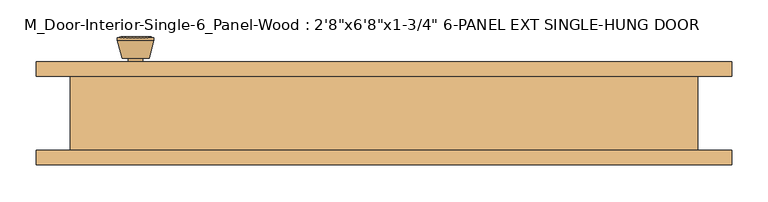
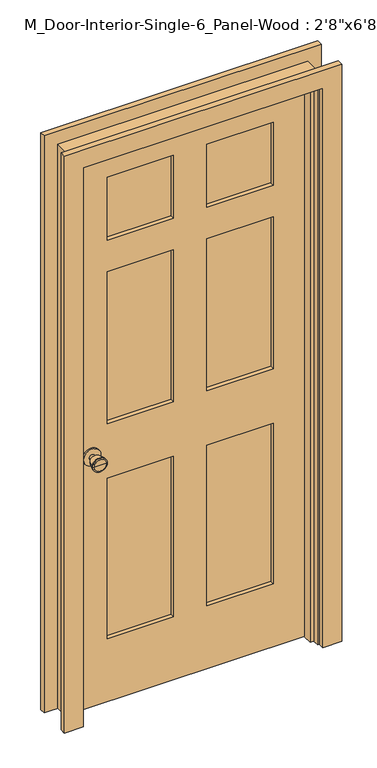
"""IFC4 building model written with IfcOpenShell, lengths in millimetres: door geometry."""

from ifc_helpers import new_model, si_unit, point, frame, frame_2d, origin, place, context, project, spatial, polyline, circle_curve, trimmed, segment, composite_curve, outline, extrude, faceted_brep, source, transform, mapped, element, save
from ifc_brep_helpers import plane_surface, cylinder_surface, revolved_surface, advanced_brep


def door_1e006c27(model_context):
    return source(origin(), model_context, "Body", "SolidModel", [
        advanced_brep(
        [(-341.4, -2.825, 914.4), (-331.4, -2.825, 914.4), (-351.4, -2.825, 914.4), (-320.9241324, -51.825, 914.4), (-341.4, -51.825, 914.4), (-361.8758676, -51.825, 914.4), (-316.4, -49.9971319, 914.4), (-366.4, -49.9971319, 914.4), (-316.4, -46.5334537, 914.4), (-366.4, -46.5334537, 914.4), (-322.763764, -21.825, 914.4), (-360.036236, -21.825, 914.4), (-331.4, -21.825, 914.4), (-351.4, -21.825, 914.4)],
        [
            (0, 1),
            (1, 2, circle_curve(frame((-341.4, -2.825, 914.4), z_axis=(0.0, 1.0, 0.0), x_axis=(-1.0, 0.0, 0.0)), 10.0)),
            (2, 0),
            (2, 1, circle_curve(frame((-341.4, -2.825, 914.4), z_axis=(0.0, 1.0, 0.0), x_axis=(-1.0, 0.0, 0.0)), 10.0)),
            (3, 4),
            (4, 5),
            (5, 3, circle_curve(frame((-341.4, -51.825, 914.4), z_axis=(0.0, -1.0, 0.0), x_axis=(-1.0, 0.0, 0.0)), 20.4758676)),
            (3, 5, circle_curve(frame((-341.4, -51.825, 914.4), z_axis=(0.0, -1.0, 0.0), x_axis=(-1.0, 0.0, 0.0)), 20.4758676)),
            (6, 3),
            (5, 7),
            (7, 6, circle_curve(frame((-341.4, -49.9971319, 914.4), z_axis=(0.0, -1.0, 0.0), x_axis=(-1.0, 0.0, 0.0)), 25.0)),
            (6, 7, circle_curve(frame((-341.4, -49.9971319, 914.4), z_axis=(0.0, -1.0, 0.0), x_axis=(-1.0, 0.0, 0.0)), 25.0)),
            (8, 6),
            (7, 9),
            (9, 8, circle_curve(frame((-341.4, -46.5334537, 914.4), z_axis=(0.0, -1.0, 0.0), x_axis=(-1.0, 0.0, 0.0)), 25.0)),
            (8, 9, circle_curve(frame((-341.4, -46.5334537, 914.4), z_axis=(0.0, -1.0, 0.0), x_axis=(-1.0, 0.0, 0.0)), 25.0)),
            (10, 8),
            (9, 11),
            (11, 10, circle_curve(frame((-341.4, -21.825, 914.4), z_axis=(0.0, -1.0, 0.0), x_axis=(-1.0, 0.0, 0.0)), 18.636236)),
            (10, 11, circle_curve(frame((-341.4, -21.825, 914.4), z_axis=(0.0, -1.0, 0.0), x_axis=(-1.0, 0.0, 0.0)), 18.636236)),
            (12, 10),
            (11, 13),
            (13, 12, circle_curve(frame((-341.4, -21.825, 914.4), z_axis=(0.0, -1.0, 0.0), x_axis=(-1.0, 0.0, 0.0)), 10.0)),
            (12, 13, circle_curve(frame((-341.4, -21.825, 914.4), z_axis=(0.0, -1.0, 0.0), x_axis=(-1.0, 0.0, 0.0)), 10.0)),
            (1, 12),
            (13, 2),
        ],
        [
            plane_surface(frame((-341.4, -2.825, 914.4), z_axis=(0.0, 1.0, 0.0), x_axis=(-1.0, 0.0, 0.0))),
            plane_surface(frame((-341.4, -51.825, 914.4), z_axis=(0.0, -1.0, 0.0), x_axis=(-1.0, 0.0, 0.0))),
            revolved_surface(polyline([(-361.8758676, -51.825, 914.4), (-366.4, -49.9971319, 914.4)]), (-341.4, -2.825, 914.4), (0.0, 1.0, 0.0)),
            cylinder_surface(frame((-341.4, -2.825, 914.4), z_axis=(0.0, 1.0, 0.0), x_axis=(-1.0, 0.0, 0.0)), 25.0),
            revolved_surface(polyline([(-366.4, -46.5334537, 914.4), (-360.036236, -21.825, 914.4)]), (-341.4, -2.825, 914.4), (0.0, 1.0, 0.0)),
            plane_surface(frame((-341.4, -21.825, 914.4), z_axis=(0.0, 1.0, 0.0), x_axis=(-1.0, 0.0, 0.0))),
            cylinder_surface(frame((-341.4, -2.825, 914.4), z_axis=(0.0, 1.0, 0.0), x_axis=(-1.0, 0.0, 0.0)), 10.0),
        ],
        [
            (0, [[1, 2, 3]]),
            (0, [[-3, 4, -1]]),
            (1, [[5, 6, 7]]),
            (1, [[-6, -5, 8]]),
            (2, [[9, -7, 10, 11]]),
            (2, [[-10, -8, -9, 12]]),
            (3, [[13, -11, 14, 15]]),
            (3, [[-14, -12, -13, 16]]),
            (4, [[17, -15, 18, 19]]),
            (4, [[-18, -16, -17, 20]]),
            (5, [[21, -19, 22, 23]]),
            (5, [[-22, -20, -21, 24]]),
            (6, [[25, -23, 26, -2]]),
            (6, [[-26, -24, -25, -4]]),
        ],
    ),
        extrude(outline(composite_curve([segment(trimmed(circle_curve(frame_2d((914.4, -341.4)), 30.0), [point((914.4, -371.4))], [point((914.4, -311.4))], False, "CARTESIAN"), True, "CONTINUOUS"), segment(trimmed(circle_curve(frame_2d((914.4, -341.4)), 30.0), [point((914.4, -311.4))], [point((914.4, -371.4))], False, "CARTESIAN"), True, "CONTINUOUS")], self_intersect=False)), frame((0.0, -2.825, 0.0), z_axis=(0.0, 1.0, 0.0), x_axis=(0.0, 0.0, 1.0)), (0.0, 0.0, 1.0), 6.0),
        advanced_brep(
        [(-341.4, 53.625, 914.4), (-351.4, 53.625, 914.4), (-331.4, 53.625, 914.4), (-320.9241324, 102.625, 914.4), (-361.8758676, 102.625, 914.4), (-341.4, 102.625, 914.4), (-316.4, 100.7971319, 914.4), (-366.4, 100.7971319, 914.4), (-316.4, 97.3334537, 914.4), (-366.4, 97.3334537, 914.4), (-322.763764, 72.625, 914.4), (-360.036236, 72.625, 914.4), (-331.4, 72.625, 914.4), (-351.4, 72.625, 914.4)],
        [
            (0, 1),
            (1, 2, circle_curve(frame((-341.4, 53.625, 914.4), z_axis=(0.0, -1.0, 0.0), x_axis=(-1.0, 0.0, 0.0)), 10.0)),
            (2, 0),
            (2, 1, circle_curve(frame((-341.4, 53.625, 914.4), z_axis=(0.0, -1.0, 0.0), x_axis=(-1.0, 0.0, 0.0)), 10.0)),
            (3, 4, circle_curve(frame((-341.4, 102.625, 914.4), z_axis=(0.0, 1.0, 0.0), x_axis=(-1.0, 0.0, 0.0)), 20.4758676)),
            (4, 5),
            (5, 3),
            (4, 3, circle_curve(frame((-341.4, 102.625, 914.4), z_axis=(0.0, 1.0, 0.0), x_axis=(-1.0, 0.0, 0.0)), 20.4758676)),
            (6, 7, circle_curve(frame((-341.4, 100.7971319, 914.4), z_axis=(0.0, 1.0, 0.0), x_axis=(-1.0, 0.0, 0.0)), 25.0)),
            (7, 4),
            (3, 6),
            (7, 6, circle_curve(frame((-341.4, 100.7971319, 914.4), z_axis=(0.0, 1.0, 0.0), x_axis=(-1.0, 0.0, 0.0)), 25.0)),
            (8, 9, circle_curve(frame((-341.4, 97.3334537, 914.4), z_axis=(0.0, 1.0, 0.0), x_axis=(-1.0, 0.0, 0.0)), 25.0)),
            (9, 7),
            (6, 8),
            (9, 8, circle_curve(frame((-341.4, 97.3334537, 914.4), z_axis=(0.0, 1.0, 0.0), x_axis=(-1.0, 0.0, 0.0)), 25.0)),
            (10, 11, circle_curve(frame((-341.4, 72.625, 914.4), z_axis=(0.0, 1.0, 0.0), x_axis=(-1.0, 0.0, 0.0)), 18.636236)),
            (11, 9),
            (8, 10),
            (11, 10, circle_curve(frame((-341.4, 72.625, 914.4), z_axis=(0.0, 1.0, 0.0), x_axis=(-1.0, 0.0, 0.0)), 18.636236)),
            (12, 13, circle_curve(frame((-341.4, 72.625, 914.4), z_axis=(0.0, 1.0, 0.0), x_axis=(-1.0, 0.0, 0.0)), 10.0)),
            (13, 11),
            (10, 12),
            (13, 12, circle_curve(frame((-341.4, 72.625, 914.4), z_axis=(0.0, 1.0, 0.0), x_axis=(-1.0, 0.0, 0.0)), 10.0)),
            (1, 13),
            (12, 2),
        ],
        [
            plane_surface(frame((-341.4, 53.625, 914.4), z_axis=(0.0, -1.0, 0.0), x_axis=(-1.0, 0.0, 0.0))),
            plane_surface(frame((-341.4, 102.625, 914.4), z_axis=(0.0, 1.0, 0.0), x_axis=(-1.0, 0.0, 0.0))),
            revolved_surface(polyline([(-361.8758676, 102.625, 914.4), (-366.4, 100.7971319, 914.4)]), (-341.4, 53.625, 914.4), (0.0, -1.0, 0.0)),
            cylinder_surface(frame((-341.4, 53.625, 914.4), z_axis=(0.0, -1.0, 0.0), x_axis=(-1.0, 0.0, 0.0)), 25.0),
            revolved_surface(polyline([(-366.4, 97.3334537, 914.4), (-360.036236, 72.625, 914.4)]), (-341.4, 53.625, 914.4), (0.0, -1.0, 0.0)),
            plane_surface(frame((-341.4, 72.625, 914.4), z_axis=(0.0, -1.0, 0.0), x_axis=(-1.0, 0.0, 0.0))),
            cylinder_surface(frame((-341.4, 53.625, 914.4), z_axis=(0.0, -1.0, 0.0), x_axis=(-1.0, 0.0, 0.0)), 10.0),
        ],
        [
            (0, [[1, 2, 3]]),
            (0, [[-3, 4, -1]]),
            (1, [[5, 6, 7]]),
            (1, [[8, -7, -6]]),
            (2, [[9, 10, -5, 11]]),
            (2, [[12, -11, -8, -10]]),
            (3, [[13, 14, -9, 15]]),
            (3, [[16, -15, -12, -14]]),
            (4, [[17, 18, -13, 19]]),
            (4, [[20, -19, -16, -18]]),
            (5, [[21, 22, -17, 23]]),
            (5, [[24, -23, -20, -22]]),
            (6, [[-2, 25, -21, 26]]),
            (6, [[-4, -26, -24, -25]]),
        ],
    ),
        extrude(outline(composite_curve([segment(trimmed(circle_curve(frame_2d((914.4, -341.4)), 30.0), [point((914.4, -371.4))], [point((914.4, -311.4))], False, "CARTESIAN"), True, "CONTINUOUS"), segment(trimmed(circle_curve(frame_2d((914.4, -341.4)), 30.0), [point((914.4, -311.4))], [point((914.4, -371.4))], False, "CARTESIAN"), True, "CONTINUOUS")], self_intersect=False)), frame((0.0, 47.625, 0.0), z_axis=(0.0, 1.0, 0.0), x_axis=(0.0, 0.0, 1.0)), (0.0, 0.0, 1.0), 6.0),
        extrude(outline(polyline([(286.4, 17.9916667), (57.5, 17.9916667), (57.5, 32.8083333), (286.4, 32.8083333), (286.4, 17.9916667)])), frame((0.0, 0.0, 1683.1), z_axis=(0.0, 0.0, 1.0), x_axis=(1.0, 0.0, 0.0)), (0.0, 0.0, 1.0), 228.9),
        extrude(outline(polyline([(286.4, 17.9916667), (57.5, 17.9916667), (57.5, 32.8083333), (286.4, 32.8083333), (286.4, 17.9916667)])), frame((0.0, 0.0, 1014.4), z_axis=(0.0, 0.0, 1.0), x_axis=(1.0, 0.0, 0.0)), (0.0, 0.0, 1.0), 553.7),
        extrude(outline(polyline([(-57.5, 17.9916667), (-286.4, 17.9916667), (-286.4, 32.8083333), (-57.5, 32.8083333), (-57.5, 17.9916667)])), frame((0.0, 0.0, 1014.4), z_axis=(0.0, 0.0, 1.0), x_axis=(1.0, 0.0, 0.0)), (0.0, 0.0, 1.0), 553.7),
        extrude(outline(polyline([(-57.5, 17.9916667), (-286.4, 17.9916667), (-286.4, 32.8083333), (-57.5, 32.8083333), (-57.5, 17.9916667)])), frame((0.0, 0.0, 1683.1), z_axis=(0.0, 0.0, 1.0), x_axis=(1.0, 0.0, 0.0)), (0.0, 0.0, 1.0), 228.9),
        extrude(outline(polyline([(286.4, 17.9916667), (57.5, 17.9916667), (57.5, 32.8083333), (286.4, 32.8083333), (286.4, 17.9916667)])), frame((0.0, 0.0, 230.0), z_axis=(0.0, 0.0, 1.0), x_axis=(1.0, 0.0, 0.0)), (0.0, 0.0, 1.0), 584.4),
        extrude(outline(polyline([(-57.5, 17.9916667), (-286.4, 17.9916667), (-286.4, 32.8083333), (-57.5, 32.8083333), (-57.5, 17.9916667)])), frame((0.0, 0.0, 230.0), z_axis=(0.0, 0.0, 1.0), x_axis=(1.0, 0.0, 0.0)), (0.0, 0.0, 1.0), 584.4),
        extrude(outline(polyline([(2032.0, -406.4), (0.0, -406.4), (0.0, 406.4), (2032.0, 406.4), (2032.0, -406.4)]), holes=[polyline([(1912.0, 57.5), (1912.0, 286.4), (1683.1, 286.4), (1683.1, 57.5), (1912.0, 57.5)]), polyline([(1568.1, 286.4), (1014.4, 286.4), (1014.4, 57.5), (1568.1, 57.5), (1568.1, 286.4)]), polyline([(1014.4, -57.5), (1014.4, -286.4), (1568.1, -286.4), (1568.1, -57.5), (1014.4, -57.5)]), polyline([(1683.1, -286.4), (1912.0, -286.4), (1912.0, -57.5), (1683.1, -57.5), (1683.1, -286.4)]), polyline([(814.4, 57.5), (814.4, 286.4), (230.0, 286.4), (230.0, 57.5), (814.4, 57.5)]), polyline([(230.0, -57.5), (230.0, -286.4), (814.4, -286.4), (814.4, -57.5), (230.0, -57.5)])]), frame((0.0, 3.175, 0.0), z_axis=(0.0, 1.0, 0.0), x_axis=(0.0, 0.0, 1.0)), (0.0, 0.0, 1.0), 44.45),
        faceted_brep([(431.4, 47.625, 0.0), (431.4, -53.975, 0.0), (406.4, -53.975, 0.0), (406.4, -31.75, 0.0), (393.7, -31.75, 0.0), (393.7, 3.175, 0.0), (406.4, 3.175, 0.0), (406.4, 47.625, 0.0), (431.4, 47.625, 2057.0), (431.4, -53.975, 2057.0), (-431.4, -53.975, 2057.0), (-431.4, -53.975, 0.0), (-406.4, -53.975, 0.0), (-406.4, -53.975, 2032.0), (406.4, -53.975, 2032.0), (406.4, -31.75, 2032.0), (-406.4, -31.75, 2032.0), (-406.4, -31.75, 0.0), (-393.7, -31.75, 0.0), (-393.7, -31.75, 2019.3), (393.7, -31.75, 2019.3), (393.7, 3.175, 2019.3), (-393.7, 3.175, 2019.3), (-393.7, 3.175, 0.0), (-406.4, 3.175, 0.0), (-406.4, 3.175, 2032.0), (406.4, 3.175, 2032.0), (406.4, 47.625, 2032.0), (-406.4, 47.625, 2032.0), (-406.4, 47.625, 0.0), (-431.4, 47.625, 0.0), (-431.4, 47.625, 2057.0)], [[[0, 1, 2, 3, 4, 5, 6, 7]], [[1, 0, 8, 9]], [[2, 1, 9, 10, 11, 12, 13, 14]], [[3, 2, 14, 15]], [[4, 3, 15, 16, 17, 18, 19, 20]], [[5, 4, 20, 21]], [[6, 5, 21, 22, 23, 24, 25, 26]], [[7, 6, 26, 27]], [[0, 7, 27, 28, 29, 30, 31, 8]], [[9, 8, 31, 10]], [[15, 14, 13, 16]], [[21, 20, 19, 22]], [[27, 26, 25, 28]], [[30, 29, 24, 23, 18, 17, 12, 11]], [[10, 31, 30, 11]], [[16, 13, 12, 17]], [[22, 19, 18, 23]], [[28, 25, 24, 29]]]),
        extrude(outline(polyline([(0.0, 412.75), (0.0, 477.75), (2103.35, 477.75), (2103.35, -477.75), (0.0, -477.75), (0.0, -412.75), (2038.35, -412.75), (2038.35, 412.75), (0.0, 412.75)])), frame((0.0, -73.975, 0.0), z_axis=(0.0, 1.0, 0.0), x_axis=(0.0, 0.0, 1.0)), (0.0, 0.0, 1.0), 20.0),
        extrude(outline(polyline([(0.0, 412.75), (0.0, 477.75), (2103.35, 477.75), (2103.35, -477.75), (0.0, -477.75), (0.0, -412.75), (2038.35, -412.75), (2038.35, 412.75), (0.0, 412.75)])), frame((0.0, 47.625, 0.0), z_axis=(0.0, 1.0, 0.0), x_axis=(0.0, 0.0, 1.0)), (0.0, 0.0, 1.0), 20.0),
    ])


if __name__ == "__main__":
    model = new_model("IFC4")
    model_context = context("Model", 3, world=origin())
    ifc_project = project(units=[si_unit("LENGTHUNIT", "METRE", prefix="MILLI")], contexts=[model_context])
    site = spatial("IfcSite", under=ifc_project)
    building = spatial("IfcBuilding", under=site)
    placement = place(None, origin())
    door_shape = door_1e006c27(model_context)
    element("IfcDoor", 1, ObjectType="M_Door-Interior-Single-6_Panel-Wood : 2'8\"x6'8\"x1-3/4\" 6-PANEL EXT SINGLE-HUNG DOOR", at=placement, inside=building, context=model_context, shape_type="MappedRepresentation", body=[
        mapped(door_shape, transform((0.0, 0.0, 0.0), x_axis=(1.0, 0.0, 0.0), y_axis=(0.0, 1.0, 0.0), z_axis=(0.0, 0.0, 1.0))),
    ])
    save(model, "model.ifc")

# Revit data of these elements
# Type "M_Door-Interior-Single-6_Panel-Wood : 2'8\"x6'8\"x1-3/4\" 6-PANEL EXT SINGLE-HUNG DOOR"
#   Type Mark = "37"
#   Assembly Code = "C1020300"
#   Analytic Construction = "Wooden"
#   Top Rail = 0' - 4.72441"
#   Top Panel = 0' - 9.01181"
#   Thickness = 0' - 1 3/4"
#   Thermal Resistance (R) = 2.5876 (h·ft²·°F)/BTU
#   Swing Angle [instance default] = 90.00°
#   Stiles = 0' - 4.72441"
#   Rough Width = 2' - 9.9685"
#   Rough Height = 6' - 8.98425"
#   Mullion = 0' - 4.52756"
#   Lock Rail = 0' - 7.87402"
#   Intermediate Rail = 0' - 4.52756"
#   Height = 6' - 8"
#   Width = 2' - 8"
#   Heat Transfer Coefficient (U) = 0.3865 BTU/(h·ft²·°F)
#   Bottom Rail = 0' - 9.05512"
#   Trim Material = Cherry
#   Panel Material = Cherry
#   Frame Material = Cherry
#   Door Handle Material = Aluminum
#   Visual Light Transmittance = 0
#   Solar Heat Gain Coefficient = 0
#   Wall Closure = (empty or 0)
#   Function = (empty or 0)
# Element 1 (IfcDoor, "M_Door-Interior-Single-6_Panel-Wood : 2'8\"x6'8\"x1-3/4\" 6-PANEL EXT SINGLE-HUNG DOOR")
#   Materials on its faces: "Cherry", "Aluminum"
# Materials
#   "Cherry": class "Wood", colour RGB 226 177 128, transparency 0, Description = "Prunus Serotina", Cost = 0
#   "Aluminum": class "Metal", colour RGB 244 244 244, transparency 0, Description = "Aluminum 6061", Cost = 0
